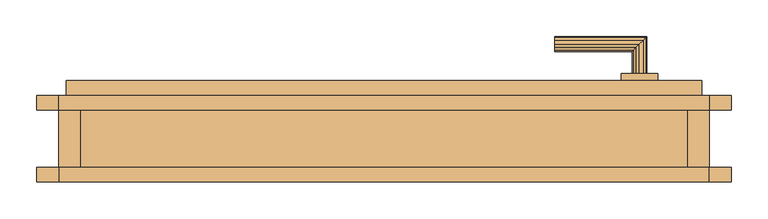
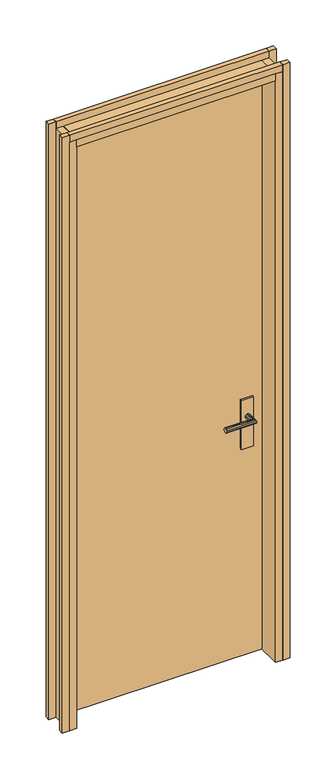
"""IFC4 building model written with IfcOpenShell, lengths in millimetres: door geometry, Tür."""

from ifc_helpers import new_model, si_unit, frame, origin, place, context, project, spatial, polyline, outline, extrude, faceted_brep, source, transform, mapped, element, save


def door_aaf3adaa(model_context):
    return source(origin(), model_context, "Body", "SolidModel", [
        faceted_brep([(795.0, 128.0, 1198.660254), (790.0, 128.0, 1200.0), (785.0, 128.0, 1198.660254), (781.339746, 128.0, 1195.0), (780.0, 128.0, 1190.0), (781.339746, 128.0, 1185.0), (785.0, 128.0, 1181.339746), (790.0, 128.0, 1180.0), (795.0, 128.0, 1181.339746), (798.660254, 128.0, 1185.0), (800.0, 128.0, 1190.0), (798.660254, 128.0, 1195.0), (790.0, 168.0, 1200.0), (795.0, 173.0, 1198.660254), (798.660254, 176.660254, 1195.0), (800.0, 178.0, 1190.0), (798.660254, 176.660254, 1185.0), (795.0, 173.0, 1181.339746), (790.0, 168.0, 1180.0), (785.0, 163.0, 1181.339746), (781.339746, 159.339746, 1185.0), (780.0, 158.0, 1190.0), (781.339746, 159.339746, 1195.0), (785.0, 163.0, 1198.660254), (675.0, 163.0, 1198.660254), (675.0, 168.0, 1200.0), (675.0, 173.0, 1198.660254), (675.0, 176.660254, 1195.0), (675.0, 178.0, 1190.0), (675.0, 176.660254, 1185.0), (675.0, 173.0, 1181.339746), (675.0, 168.0, 1180.0), (675.0, 163.0, 1181.339746), (675.0, 159.339746, 1185.0), (675.0, 158.0, 1190.0), (675.0, 159.339746, 1195.0)], [[[0, 1, 2, 3, 4, 5, 6, 7, 8, 9, 10, 11]], [[12, 1, 0, 13]], [[13, 0, 11, 14]], [[14, 11, 10, 15]], [[15, 10, 9, 16]], [[16, 9, 8, 17]], [[17, 8, 7, 18]], [[18, 7, 6, 19]], [[19, 6, 5, 20]], [[20, 5, 4, 21]], [[21, 4, 3, 22]], [[22, 3, 2, 23]], [[23, 2, 1, 12]], [[24, 25, 26, 27, 28, 29, 30, 31, 32, 33, 34, 35]], [[25, 12, 13, 26]], [[26, 13, 14, 27]], [[27, 14, 15, 28]], [[28, 15, 16, 29]], [[29, 16, 17, 30]], [[30, 17, 18, 31]], [[31, 18, 19, 32]], [[32, 19, 20, 33]], [[33, 20, 21, 34]], [[34, 21, 22, 35]], [[35, 22, 23, 24]], [[24, 23, 12, 25]]]),
        extrude(outline(polyline([(855.0, 98.0), (855.0, -20.0), (30.0, -20.0), (30.0, 98.0), (855.0, 98.0)])), frame((0.0, 0.0, 2690.0), z_axis=(0.0, 0.0, 1.0), x_axis=(1.0, 0.0, 0.0)), (0.0, 0.0, 1.0), 30.0),
        extrude(outline(polyline([(30.0, 98.0), (30.0, -20.0), (0.0, -20.0), (0.0, 98.0), (30.0, 98.0)])), frame((0.0, 0.0, 140.0), z_axis=(0.0, 0.0, 1.0), x_axis=(1.0, 0.0, 0.0)), (0.0, 0.0, 1.0), 2580.0),
        extrude(outline(polyline([(885.0, 98.0), (885.0, 78.0), (0.0, 78.0), (0.0, 98.0), (885.0, 98.0)])), frame((0.0, 0.0, 2720.0), z_axis=(0.0, 0.0, 1.0), x_axis=(1.0, 0.0, 0.0)), (0.0, 0.0, 1.0), 30.0),
        extrude(outline(polyline([(0.0, 78.0), (-30.0, 78.0), (-30.0, 98.0), (0.0, 98.0), (0.0, 78.0)])), frame((0.0, 0.0, 140.0), z_axis=(0.0, 0.0, 1.0), x_axis=(1.0, 0.0, 0.0)), (0.0, 0.0, 1.0), 2610.0),
        extrude(outline(polyline([(0.0, -20.0), (-30.0, -20.0), (-30.0, 0.0), (0.0, 0.0), (0.0, -20.0)])), frame((0.0, 0.0, 140.0), z_axis=(0.0, 0.0, 1.0), x_axis=(1.0, 0.0, 0.0)), (0.0, 0.0, 1.0), 2610.0),
        extrude(outline(polyline([(875.0, 118.0), (875.0, 78.0), (10.0, 78.0), (10.0, 118.0), (875.0, 118.0)])), frame((0.0, 0.0, 140.0), z_axis=(0.0, 0.0, 1.0), x_axis=(1.0, 0.0, 0.0)), (0.0, 0.0, 1.0), 2570.0),
        faceted_brep([(785.0, 68.0, 1198.660254), (790.0, 68.0, 1200.0), (795.0, 68.0, 1198.660254), (798.660254, 68.0, 1195.0), (800.0, 68.0, 1190.0), (798.660254, 68.0, 1185.0), (795.0, 68.0, 1181.339746), (790.0, 68.0, 1180.0), (785.0, 68.0, 1181.339746), (781.339746, 68.0, 1185.0), (780.0, 68.0, 1190.0), (781.339746, 68.0, 1195.0), (790.0, 28.0, 1200.0), (795.0, 23.0, 1198.660254), (798.660254, 19.339746, 1195.0), (800.0, 18.0, 1190.0), (798.660254, 19.339746, 1185.0), (795.0, 23.0, 1181.339746), (790.0, 28.0, 1180.0), (785.0, 33.0, 1181.339746), (781.339746, 36.660254, 1185.0), (780.0, 38.0, 1190.0), (781.339746, 36.660254, 1195.0), (785.0, 33.0, 1198.660254), (675.0, 23.0, 1198.660254), (675.0, 28.0, 1200.0), (675.0, 33.0, 1198.660254), (675.0, 36.660254, 1195.0), (675.0, 38.0, 1190.0), (675.0, 36.660254, 1185.0), (675.0, 33.0, 1181.339746), (675.0, 28.0, 1180.0), (675.0, 23.0, 1181.339746), (675.0, 19.339746, 1185.0), (675.0, 18.0, 1190.0), (675.0, 19.339746, 1195.0)], [[[0, 1, 2, 3, 4, 5, 6, 7, 8, 9, 10, 11]], [[2, 1, 12, 13]], [[3, 2, 13, 14]], [[4, 3, 14, 15]], [[5, 4, 15, 16]], [[6, 5, 16, 17]], [[7, 6, 17, 18]], [[8, 7, 18, 19]], [[9, 8, 19, 20]], [[10, 9, 20, 21]], [[11, 10, 21, 22]], [[0, 11, 22, 23]], [[1, 0, 23, 12]], [[24, 25, 26, 27, 28, 29, 30, 31, 32, 33, 34, 35]], [[13, 12, 25, 24]], [[14, 13, 24, 35]], [[15, 14, 35, 34]], [[16, 15, 34, 33]], [[17, 16, 33, 32]], [[18, 17, 32, 31]], [[19, 18, 31, 30]], [[20, 19, 30, 29]], [[21, 20, 29, 28]], [[22, 21, 28, 27]], [[23, 22, 27, 26]], [[12, 23, 26, 25]]]),
        extrude(outline(polyline([(915.0, 0.0), (915.0, -20.0), (885.0, -20.0), (885.0, 0.0), (915.0, 0.0)])), frame((0.0, 0.0, 140.0), z_axis=(0.0, 0.0, 1.0), x_axis=(1.0, 0.0, 0.0)), (0.0, 0.0, 1.0), 2610.0),
        extrude(outline(polyline([(885.0, 98.0), (885.0, -20.0), (855.0, -20.0), (855.0, 98.0), (885.0, 98.0)])), frame((0.0, 0.0, 140.0), z_axis=(0.0, 0.0, 1.0), x_axis=(1.0, 0.0, 0.0)), (0.0, 0.0, 1.0), 2580.0),
        extrude(outline(polyline([(915.0, 98.0), (915.0, 78.0), (885.0, 78.0), (885.0, 98.0), (915.0, 98.0)])), frame((0.0, 0.0, 140.0), z_axis=(0.0, 0.0, 1.0), x_axis=(1.0, 0.0, 0.0)), (0.0, 0.0, 1.0), 2610.0),
        extrude(outline(polyline([(815.0, 128.0), (815.0, 118.0), (765.0, 118.0), (765.0, 128.0), (815.0, 128.0)])), frame((0.0, 0.0, 1050.0), z_axis=(0.0, 0.0, 1.0), x_axis=(1.0, 0.0, 0.0)), (0.0, 0.0, 1.0), 215.0),
        extrude(outline(polyline([(885.0, 0.0), (885.0, -20.0), (0.0, -20.0), (0.0, 0.0), (885.0, 0.0)])), frame((0.0, 0.0, 2720.0), z_axis=(0.0, 0.0, 1.0), x_axis=(1.0, 0.0, 0.0)), (0.0, 0.0, 1.0), 30.0),
        extrude(outline(polyline([(765.0, 78.0), (815.0, 78.0), (815.0, 68.0), (765.0, 68.0), (765.0, 78.0)])), frame((0.0, 0.0, 1050.0), z_axis=(0.0, 0.0, 1.0), x_axis=(1.0, 0.0, 0.0)), (0.0, 0.0, 1.0), 215.0),
    ])


if __name__ == "__main__":
    model = new_model("IFC4")
    model_context = context("Model", 3, world=origin())
    ifc_project = project(units=[si_unit("LENGTHUNIT", "METRE", prefix="MILLI")], contexts=[model_context])
    site = spatial("IfcSite", under=ifc_project)
    building = spatial("IfcBuilding", under=site)
    placement = place(None, origin())
    door_shape = door_aaf3adaa(model_context)
    element("IfcDoor", 1, ObjectType="Tür", at=placement, inside=building, context=model_context, shape_type="MappedRepresentation", body=[
        mapped(door_shape, transform((0.0, 0.0, 0.0), x_axis=(1.0, 0.0, 0.0), y_axis=(0.0, 1.0, 0.0), z_axis=(0.0, 0.0, 1.0))),
    ])
    save(model, "model.ifc")

# Revit data of these elements
# Type "Tür"
#   Type Mark = "62"
# Element 1 (IfcDoor, "Tür")
#   Materials on its faces: "tuer_beschlag", "tuer_holzzarge"
# Materials
#   "tuer_beschlag": class "Unassigned", colour RGB 128 128 128, transparency 0
#   "tuer_holzzarge": class "Unassigned", colour RGB 255 255 255, transparency 0
